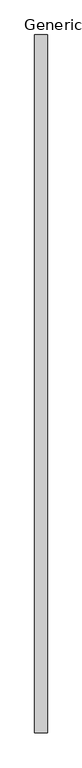
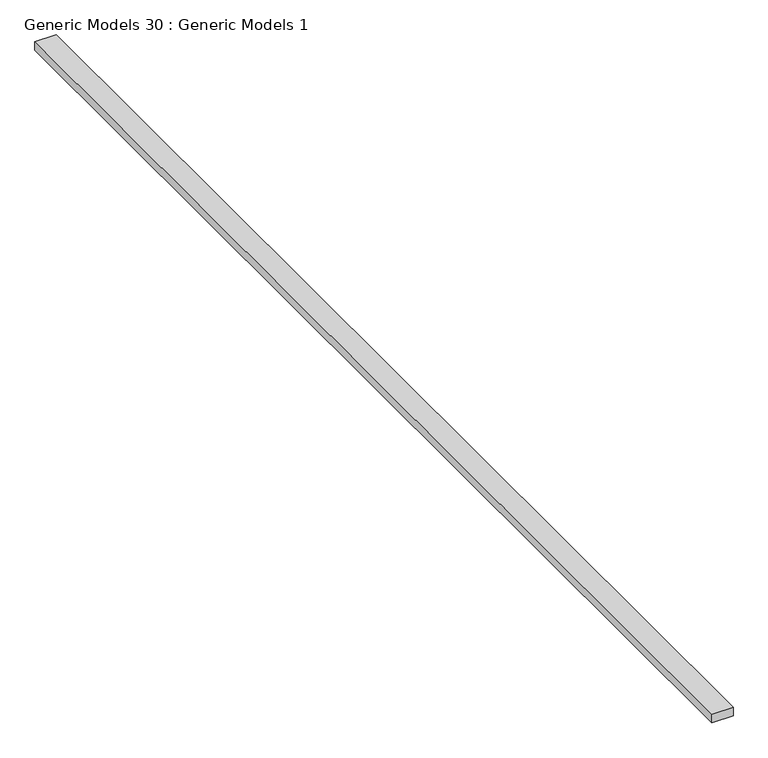
"""IFC4 building model written with IfcOpenShell, lengths in millimetres: proxy geometry, Generic Models 30 : Generic Models 1."""

from ifc_helpers import new_model, si_unit, frame, origin, place, context, project, spatial, polyline, outline, extrude, source, transform, mapped, element, save


def generic_models_30_generic_models_1_4e067135(model_context):
    return source(origin(), model_context, "Body", "SweptSolid", [
        extrude(outline(polyline([(-9207.6736295, 11981.8769662), (-9118.7736295, 11981.8769662), (-9118.7736295, 7054.2769662), (-9207.6736295, 7054.2769662), (-9207.6736295, 11981.8769662)])), frame((0.0, 0.0, 126427.2447533), z_axis=(0.0, 0.0, 1.0), x_axis=(1.0, 0.0, 0.0)), (0.0, 0.0, 1.0), 38.1),
    ])


if __name__ == "__main__":
    model = new_model("IFC4")
    model_context = context("Model", 3, world=origin())
    ifc_project = project(units=[si_unit("LENGTHUNIT", "METRE", prefix="MILLI")], contexts=[model_context])
    site = spatial("IfcSite", under=ifc_project)
    building = spatial("IfcBuilding", under=site)
    placement = place(None, origin())
    generic_models_30_generic_models_1_shape = generic_models_30_generic_models_1_4e067135(model_context)
    element("IfcBuildingElementProxy", 1, Name="Generic Models 30 : Generic Models 1", ObjectType="Generic Models 30 : Generic Models 1", at=placement, inside=building, context=model_context, shape_type="MappedRepresentation", body=[
        mapped(generic_models_30_generic_models_1_shape, transform((0.0, 0.0, 0.0), x_axis=(1.0, 0.0, 0.0), y_axis=(0.0, 1.0, 0.0), z_axis=(0.0, 0.0, 1.0))),
    ])
    save(model, "model.ifc")

# Revit data of these elements
# Element 1 (IfcBuildingElementProxy, "Generic Models 30 : Generic Models 1")
#   Materials on its faces: "_2X BLOCKING AS REQUIRED"
# Materials
#   "_2X BLOCKING AS REQUIRED": class "Generic", colour RGB 177 130 114, transparency 0, Cost = 0
